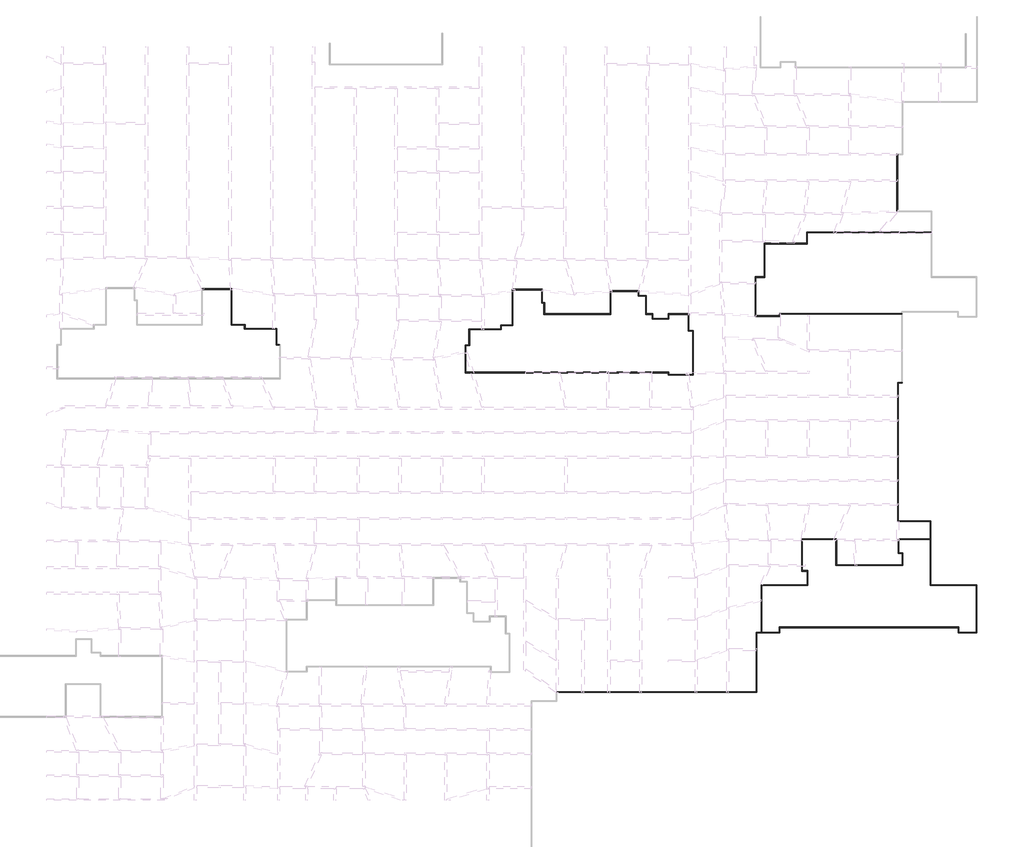
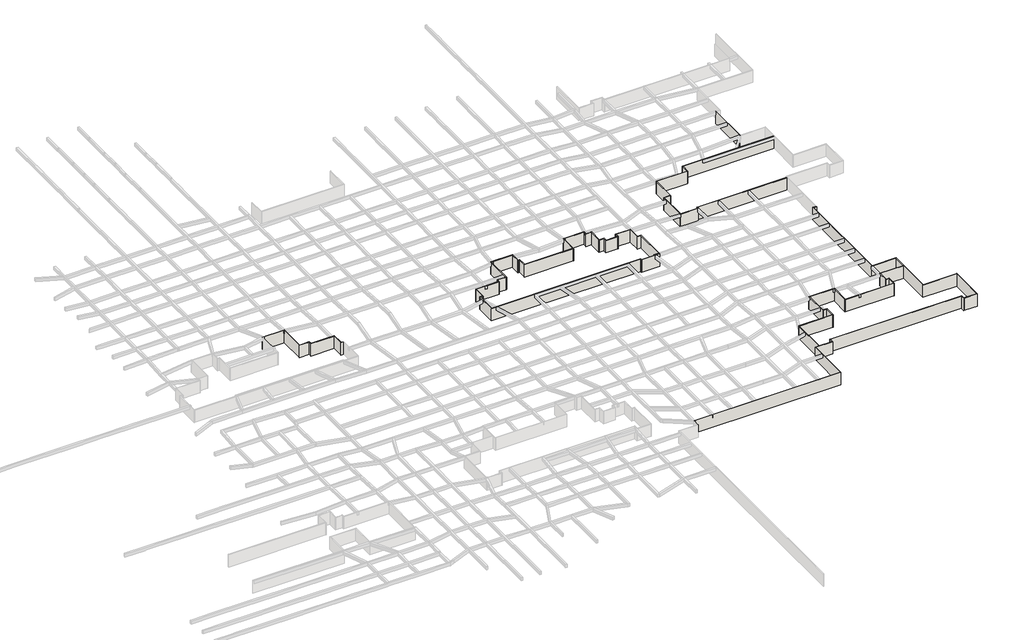
# One storey, part 4 of 45: 70 walls.
"""IFC4 building model written with IfcOpenShell, lengths in millimetres."""

from ifc_helpers import new_model, si_unit, origin, origin_with_axes, place, context, project, spatial, polyline, outline, extrude, faceted_brep, element, save

model = new_model("IFC4")

# Units and contexts
model_context = context("Model", 3, world=origin())
ifc_project = project(units=[si_unit("LENGTHUNIT", "METRE", prefix="MILLI")], contexts=[model_context])

# Site, building, storey
site = spatial("IfcSite", under=ifc_project)
building = spatial("IfcBuilding", under=site)
storey = spatial("IfcBuildingStorey", under=building, Name="户型图", Elevation=0.0)

# Walls
placement = place(None, origin())
element("IfcWall", 1, ObjectType="所有墙体", at=placement, inside=storey, context=model_context, shape_type="Brep", body=[
    faceted_brep([(-180.5216564, -109988.0123265, 0.0), (37119.4783436, -109988.0123265, 0.0), (37119.4783436, -109988.0123265, 3300.0), (-180.5216564, -109988.0123265, 3300.0), (-180.5216564, -109868.0123265, 0.0), (-180.5216564, -109868.0123265, 3300.0), (36999.4783436, -109868.0123265, 3300.0), (37119.4783436, -109868.0123265, 3300.0), (37119.4783436, -109868.0123265, 0.0), (36999.4783436, -109868.0123265, 0.0)], [[[0, 1, 2, 3]], [[4, 5, 6, 7, 8, 9]], [[1, 0, 4, 9, 8]], [[3, 2, 7, 6, 5]], [[0, 3, 5, 4]], [[2, 1, 8, 7]]]),
])
element("IfcWall", 2, ObjectType="所有墙体", at=placement, inside=storey, context=model_context, shape_type="Brep", body=[
    faceted_brep([(37119.4783436, -109868.0123265, 0.0), (37119.4783436, -98888.0123265, 0.0), (37119.4783436, -98768.0123265, 0.0), (37119.4783436, -98768.0123265, 3300.0), (37119.4783436, -98888.0123265, 3300.0), (37119.4783436, -109868.0123265, 3300.0), (36999.4783436, -109868.0123265, 0.0), (36999.4783436, -109868.0123265, 3300.0), (36999.4783436, -98768.0123265, 3300.0), (36999.4783436, -98768.0123265, 0.0)], [[[0, 1, 2, 3, 4, 5]], [[6, 7, 8, 9]], [[2, 1, 0, 6, 9]], [[5, 4, 3, 8, 7]], [[0, 5, 7, 6]], [[3, 2, 9, 8]]]),
])
element("IfcWall", 3, ObjectType="所有墙体", at=placement, inside=storey, context=model_context, shape_type="Brep", body=[
    faceted_brep([(37119.4783436, -98888.0123265, 0.0), (41419.4783436, -98888.0123265, 0.0), (41419.4783436, -98888.0123265, 3300.0), (37119.4783436, -98888.0123265, 3300.0), (37119.4783436, -98768.0123265, 0.0), (37119.4783436, -98768.0123265, 3300.0), (37945.7968791, -98768.0123265, 3300.0), (38065.7968791, -98768.0123265, 3300.0), (41299.4783436, -98768.0123265, 3300.0), (41419.4783436, -98768.0123265, 3300.0), (41419.4783436, -98768.0123265, 0.0), (41299.4783436, -98768.0123265, 0.0), (38065.7968791, -98768.0123265, 0.0), (37945.7968791, -98768.0123265, 0.0)], [[[0, 1, 2, 3]], [[4, 5, 6, 7, 8, 9, 10, 11, 12, 13]], [[1, 0, 4, 13, 12, 11, 10]], [[3, 2, 9, 8, 7, 6, 5]], [[0, 3, 5, 4]], [[2, 1, 10, 9]]]),
])
element("IfcWall", 4, ObjectType="所有墙体", at=placement, inside=storey, context=model_context, shape_type="Brep", body=[
    faceted_brep([(41419.4783436, -98768.0123265, 0.0), (41419.4783436, -97888.0123265, 0.0), (41419.4783436, -97768.0123265, 0.0), (41419.4783436, -97768.0123265, 3300.0), (41419.4783436, -97888.0123265, 3300.0), (41419.4783436, -98768.0123265, 3300.0), (41299.4783436, -98768.0123265, 0.0), (41299.4783436, -98768.0123265, 3300.0), (41299.4783436, -97768.0123265, 3300.0), (41299.4783436, -97768.0123265, 0.0)], [[[0, 1, 2, 3, 4, 5]], [[6, 7, 8, 9]], [[2, 1, 0, 6, 9]], [[5, 4, 3, 8, 7]], [[0, 5, 7, 6]], [[3, 2, 9, 8]]]),
])
element("IfcWall", 5, ObjectType="所有墙体", at=placement, inside=storey, context=model_context, shape_type="Brep", body=[
    faceted_brep([(41419.4783436, -97888.0123265, 0.0), (74699.4783436, -97888.0123265, 0.0), (74819.4783436, -97888.0123265, 0.0), (74819.4783436, -97888.0123265, 3300.0), (74699.4783436, -97888.0123265, 3300.0), (41419.4783436, -97888.0123265, 3300.0), (41419.4783436, -97768.0123265, 0.0), (41419.4783436, -97768.0123265, 3300.0), (74819.4783436, -97768.0123265, 3300.0), (74819.4783436, -97768.0123265, 0.0)], [[[0, 1, 2, 3, 4, 5]], [[6, 7, 8, 9]], [[2, 1, 0, 6, 9]], [[5, 4, 3, 8, 7]], [[0, 5, 7, 6]], [[3, 2, 9, 8]]]),
])
element("IfcWall", 6, ObjectType="所有墙体", at=placement, inside=storey, context=model_context, shape_type="Brep", body=[
    faceted_brep([(74699.4783436, -97888.0123265, 0.0), (74699.4783436, -98888.0123265, 0.0), (74699.4783436, -98888.0123265, 3300.0), (74699.4783436, -97888.0123265, 3300.0), (74819.4783436, -97888.0123265, 0.0), (74819.4783436, -97888.0123265, 3300.0), (74819.4783436, -98768.0123265, 3300.0), (74819.4783436, -98888.0123265, 3300.0), (74819.4783436, -98888.0123265, 0.0), (74819.4783436, -98768.0123265, 0.0)], [[[0, 1, 2, 3]], [[4, 5, 6, 7, 8, 9]], [[1, 0, 4, 9, 8]], [[3, 2, 7, 6, 5]], [[0, 3, 5, 4]], [[2, 1, 8, 7]]]),
])
element("IfcWall", 7, ObjectType="所有墙体", at=placement, inside=storey, context=model_context, shape_type="Brep", body=[
    faceted_brep([(74819.4783436, -98888.0123265, 0.0), (78219.4783436, -98888.0123265, 0.0), (78219.4783436, -98888.0123265, 3300.0), (74819.4783436, -98888.0123265, 3300.0), (74819.4783436, -98768.0123265, 0.0), (74819.4783436, -98768.0123265, 3300.0), (78099.4783436, -98768.0123265, 3300.0), (78219.4783436, -98768.0123265, 3300.0), (78219.4783436, -98768.0123265, 0.0), (78099.4783436, -98768.0123265, 0.0)], [[[0, 1, 2, 3]], [[4, 5, 6, 7, 8, 9]], [[1, 0, 4, 9, 8]], [[3, 2, 7, 6, 5]], [[0, 3, 5, 4]], [[2, 1, 8, 7]]]),
])
element("IfcWall", 8, ObjectType="所有墙体", at=placement, inside=storey, context=model_context, shape_type="Brep", body=[
    faceted_brep([(78219.4783436, -98768.0123265, 0.0), (78219.4783436, -89868.0123265, 0.0), (78219.4783436, -89868.0123265, 3300.0), (78219.4783436, -98768.0123265, 3300.0), (78099.4783436, -98768.0123265, 0.0), (78099.4783436, -98768.0123265, 3300.0), (78099.4783436, -89988.0123265, 3300.0), (78099.4783436, -89868.0123265, 3300.0), (78099.4783436, -89868.0123265, 0.0), (78099.4783436, -89988.0123265, 0.0)], [[[0, 1, 2, 3]], [[4, 5, 6, 7, 8, 9]], [[1, 0, 4, 9, 8]], [[3, 2, 7, 6, 5]], [[0, 3, 5, 4]], [[2, 1, 8, 7]]]),
])
element("IfcWall", 9, ObjectType="所有墙体", at=placement, inside=storey, context=model_context, shape_type="Brep", body=[
    faceted_brep([(78099.4783436, -89868.0123265, 0.0), (69619.4783436, -89868.0123265, 0.0), (69499.4783436, -89868.0123265, 0.0), (69499.4783436, -89868.0123265, 3300.0), (69619.4783436, -89868.0123265, 3300.0), (78099.4783436, -89868.0123265, 3300.0), (78099.4783436, -89988.0123265, 0.0), (78099.4783436, -89988.0123265, 3300.0), (69499.4783436, -89988.0123265, 3300.0), (69499.4783436, -89988.0123265, 0.0)], [[[0, 1, 2, 3, 4, 5]], [[6, 7, 8, 9]], [[2, 1, 0, 6, 9]], [[5, 4, 3, 8, 7]], [[0, 5, 7, 6]], [[3, 2, 9, 8]]]),
])
element("IfcWall", 10, ObjectType="所有墙体", at=placement, inside=storey, context=model_context, shape_type="Brep", body=[
    faceted_brep([(69619.4783436, -89868.0123265, 0.0), (69619.4783436, -77968.0123265, 0.0), (69619.4783436, -77968.0123265, 3300.0), (69619.4783436, -89868.0123265, 3300.0), (69499.4783436, -89868.0123265, 0.0), (69499.4783436, -89868.0123265, 3300.0), (69499.4783436, -81448.0123265, 3300.0), (69499.4783436, -81328.0123265, 3300.0), (69499.4783436, -78088.0123265, 3300.0), (69499.4783436, -77968.0123265, 3300.0), (69499.4783436, -77968.0123265, 0.0), (69499.4783436, -78088.0123265, 0.0), (69499.4783436, -81328.0123265, 0.0), (69499.4783436, -81448.0123265, 0.0)], [[[0, 1, 2, 3]], [[4, 5, 6, 7, 8, 9, 10, 11, 12, 13]], [[1, 0, 4, 13, 12, 11, 10]], [[3, 2, 9, 8, 7, 6, 5]], [[0, 3, 5, 4]], [[2, 1, 10, 9]]]),
])
element("IfcWall", 11, ObjectType="所有墙体", at=placement, inside=storey, context=model_context, shape_type="Brep", body=[
    faceted_brep([(69499.4783436, -77968.0123265, 0.0), (63519.4783436, -77968.0123265, 0.0), (63399.4783436, -77968.0123265, 0.0), (63399.4783436, -77968.0123265, 3300.0), (63519.4783436, -77968.0123265, 3300.0), (69499.4783436, -77968.0123265, 3300.0), (69499.4783436, -78088.0123265, 0.0), (69499.4783436, -78088.0123265, 3300.0), (63399.4783436, -78088.0123265, 3300.0), (63399.4783436, -78088.0123265, 0.0)], [[[0, 1, 2, 3, 4, 5]], [[6, 7, 8, 9]], [[2, 1, 0, 6, 9]], [[5, 4, 3, 8, 7]], [[0, 5, 7, 6]], [[3, 2, 9, 8]]]),
])
element("IfcWall", 12, ObjectType="所有墙体", at=placement, inside=storey, context=model_context, shape_type="Brep", body=[
    faceted_brep([(63519.4783436, -77968.0123265, 0.0), (63519.4783436, -52188.0123265, 0.0), (63519.4783436, -52068.0123265, 0.0), (63519.4783436, -52068.0123265, 3300.0), (63519.4783436, -52188.0123265, 3300.0), (63519.4783436, -77968.0123265, 3300.0), (63399.4783436, -77968.0123265, 0.0), (63399.4783436, -77968.0123265, 3300.0), (63399.4783436, -52068.0123265, 3300.0), (63399.4783436, -52068.0123265, 0.0)], [[[0, 1, 2, 3, 4, 5]], [[6, 7, 8, 9]], [[2, 1, 0, 6, 9]], [[5, 4, 3, 8, 7]], [[0, 5, 7, 6]], [[3, 2, 9, 8]]]),
])
element("IfcWall", 13, ObjectType="所有墙体", at=placement, inside=storey, context=model_context, shape_type="Brep", body=[
    faceted_brep([(63519.4783436, -52188.0123265, 0.0), (64319.4783436, -52188.0123265, 0.0), (64319.4783436, -52188.0123265, 3300.0), (63519.4783436, -52188.0123265, 3300.0), (63519.4783436, -52068.0123265, 0.0), (63519.4783436, -52068.0123265, 3300.0), (64199.4783436, -52068.0123265, 3300.0), (64319.4783436, -52068.0123265, 3300.0), (64319.4783436, -52068.0123265, 0.0), (64199.4783436, -52068.0123265, 0.0)], [[[0, 1, 2, 3]], [[4, 5, 6, 7, 8, 9]], [[1, 0, 4, 9, 8]], [[3, 2, 7, 6, 5]], [[0, 3, 5, 4]], [[2, 1, 8, 7]]]),
])
element("IfcWall", 14, ObjectType="所有墙体", at=placement, inside=storey, context=model_context, shape_type="Brep", body=[
    faceted_brep([(63419.4783436, -20068.0123265, 0.0), (63419.4783436, -9588.0123265, 0.0), (63419.4783436, -9468.0123265, 0.0), (63419.4783436, -9468.0123265, 3300.0), (63419.4783436, -9588.0123265, 3300.0), (63419.4783436, -20068.0123265, 3300.0), (63299.4783436, -20068.0123265, 0.0), (63299.4783436, -20068.0123265, 3300.0), (63299.4783436, -9468.0123265, 3300.0), (63299.4783436, -9468.0123265, 0.0)], [[[0, 1, 2, 3, 4, 5]], [[6, 7, 8, 9]], [[2, 1, 0, 6, 9]], [[5, 4, 3, 8, 7]], [[0, 5, 7, 6]], [[3, 2, 9, 8]]]),
])
element("IfcWall", 15, ObjectType="所有墙体", at=placement, inside=storey, context=model_context, shape_type="Brep", body=[
    faceted_brep([(69699.4783436, -24010.6851163, 0.0), (46417.7693877, -24010.6851163, 0.0), (46417.7693877, -24010.6851163, 3300.0), (69699.4783436, -24010.6851163, 3300.0), (69699.4783436, -24130.6851163, 0.0), (69699.4783436, -24130.6851163, 3300.0), (46537.7693877, -24130.6851163, 3300.0), (46417.7693877, -24130.6851163, 3300.0), (46417.7693877, -24130.6851163, 0.0), (46537.7693877, -24130.6851163, 0.0)], [[[0, 1, 2, 3]], [[4, 5, 6, 7, 8, 9]], [[1, 0, 4, 9, 8]], [[3, 2, 7, 6, 5]], [[2, 1, 8, 7]], [[0, 3, 5, 4]]]),
])
element("IfcWall", 16, ObjectType="所有墙体", at=placement, inside=storey, context=model_context, shape_type="Brep", body=[
    faceted_brep([(46417.7693877, -24130.6851163, 0.0), (46417.7693877, -26110.6851163, 0.0), (46417.7693877, -26230.6851163, 0.0), (46417.7693877, -26230.6851163, 3300.0), (46417.7693877, -26110.6851163, 3300.0), (46417.7693877, -24130.6851163, 3300.0), (46537.7693877, -24130.6851163, 0.0), (46537.7693877, -24130.6851163, 3300.0), (46537.7693877, -26230.6851163, 3300.0), (46537.7693877, -26230.6851163, 0.0)], [[[0, 1, 2, 3, 4, 5]], [[6, 7, 8, 9]], [[2, 1, 0, 6, 9]], [[5, 4, 3, 8, 7]], [[0, 5, 7, 6]], [[3, 2, 9, 8]]]),
])
element("IfcWall", 17, ObjectType="所有墙体", at=placement, inside=storey, context=model_context, shape_type="Brep", body=[
    faceted_brep([(46417.7693877, -26110.6851163, 0.0), (38517.7693877, -26110.6851163, 0.0), (38517.7693877, -26110.6851163, 3300.0), (46417.7693877, -26110.6851163, 3300.0), (46417.7693877, -26230.6851163, 0.0), (46417.7693877, -26230.6851163, 3300.0), (38637.7693877, -26230.6851163, 3300.0), (38517.7693877, -26230.6851163, 3300.0), (38517.7693877, -26230.6851163, 0.0), (38637.7693877, -26230.6851163, 0.0)], [[[0, 1, 2, 3]], [[4, 5, 6, 7, 8, 9]], [[1, 0, 4, 9, 8]], [[3, 2, 7, 6, 5]], [[0, 3, 5, 4]], [[2, 1, 8, 7]]]),
])
element("IfcWall", 18, ObjectType="所有墙体", at=placement, inside=storey, context=model_context, shape_type="Brep", body=[
    faceted_brep([(38517.7693877, -26230.6851163, 0.0), (38517.7693877, -32368.0123265, 0.0), (38517.7693877, -32488.0123265, 0.0), (38517.7693877, -32488.0123265, 3300.0), (38517.7693877, -32368.0123265, 3300.0), (38517.7693877, -26230.6851163, 3300.0), (38637.7693877, -26230.6851163, 0.0), (38637.7693877, -26230.6851163, 3300.0), (38637.7693877, -32488.0123265, 3300.0), (38637.7693877, -32488.0123265, 0.0)], [[[0, 1, 2, 3, 4, 5]], [[6, 7, 8, 9]], [[2, 1, 0, 6, 9]], [[5, 4, 3, 8, 7]], [[0, 5, 7, 6]], [[3, 2, 9, 8]]]),
])
element("IfcWall", 19, ObjectType="所有墙体", at=placement, inside=storey, context=model_context, shape_type="Brep", body=[
    faceted_brep([(38517.7693877, -32368.0123265, 0.0), (36817.7693877, -32368.0123265, 0.0), (36817.7693877, -32368.0123265, 3300.0), (38517.7693877, -32368.0123265, 3300.0), (38517.7693877, -32488.0123265, 0.0), (38517.7693877, -32488.0123265, 3300.0), (36937.7693877, -32488.0123265, 3300.0), (36817.7693877, -32488.0123265, 3300.0), (36817.7693877, -32488.0123265, 0.0), (36937.7693877, -32488.0123265, 0.0)], [[[0, 1, 2, 3]], [[4, 5, 6, 7, 8, 9]], [[1, 0, 4, 9, 8]], [[3, 2, 7, 6, 5]], [[0, 3, 5, 4]], [[2, 1, 8, 7]]]),
])
element("IfcWall", 20, ObjectType="所有墙体", at=placement, inside=storey, context=model_context, shape_type="Brep", body=[
    faceted_brep([(36817.7693877, -32488.0123265, 0.0), (36817.7693877, -39754.4925986, 0.0), (36817.7693877, -39754.4925986, 3300.0), (36817.7693877, -32488.0123265, 3300.0), (36937.7693877, -32488.0123265, 0.0), (36937.7693877, -32488.0123265, 3300.0), (36937.7693877, -39634.4925986, 3300.0), (36937.7693877, -39754.4925986, 3300.0), (36937.7693877, -39754.4925986, 0.0), (36937.7693877, -39634.4925986, 0.0)], [[[0, 1, 2, 3]], [[4, 5, 6, 7, 8, 9]], [[1, 0, 4, 9, 8]], [[3, 2, 7, 6, 5]], [[0, 3, 5, 4]], [[2, 1, 8, 7]]]),
])
element("IfcWall", 21, ObjectType="所有墙体", at=placement, inside=storey, context=model_context, shape_type="Brep", body=[
    faceted_brep([(36937.7693877, -39754.4925986, 0.0), (41406.5225603, -39754.4925986, 0.0), (41406.5225603, -39754.4925986, 3300.0), (36937.7693877, -39754.4925986, 3300.0), (36937.7693877, -39634.4925986, 0.0), (36937.7693877, -39634.4925986, 3300.0), (41286.5225603, -39634.4925986, 3300.0), (41406.5225603, -39634.4925986, 3300.0), (41406.5225603, -39634.4925986, 0.0), (41286.5225603, -39634.4925986, 0.0)], [[[0, 1, 2, 3]], [[4, 5, 6, 7, 8, 9]], [[1, 0, 4, 9, 8]], [[3, 2, 7, 6, 5]], [[0, 3, 5, 4]], [[2, 1, 8, 7]]]),
])
element("IfcWall", 22, ObjectType="所有墙体", at=placement, inside=storey, context=model_context, shape_type="Brep", body=[
    faceted_brep([(41406.5225603, -39634.4925986, 0.0), (41406.5225603, -39338.8304418, 0.0), (41406.5225603, -39218.8304418, 0.0), (41406.5225603, -39218.8304418, 3300.0), (41406.5225603, -39338.8304418, 3300.0), (41406.5225603, -39634.4925986, 3300.0), (41286.5225603, -39634.4925986, 0.0), (41286.5225603, -39634.4925986, 3300.0), (41286.5225603, -39218.8304418, 3300.0), (41286.5225603, -39218.8304418, 0.0)], [[[0, 1, 2, 3, 4, 5]], [[6, 7, 8, 9]], [[2, 1, 0, 6, 9]], [[5, 4, 3, 8, 7]], [[0, 5, 7, 6]], [[3, 2, 9, 8]]]),
])
element("IfcWall", 23, ObjectType="所有墙体", at=placement, inside=storey, context=model_context, shape_type="SweptSolid", body=[
    extrude(outline(polyline([(64199.4783436, -39338.8304418), (41406.5225603, -39338.8304418), (41406.5225603, -39218.8304418), (64199.4783436, -39218.8304418), (64199.4783436, -39338.8304418)])), origin_with_axes(), (0.0, 0.0, 1.0), 3300.0),
])
element("IfcWall", 24, ObjectType="所有墙体", at=placement, inside=storey, context=model_context, shape_type="Brep", body=[
    faceted_brep([(-17290.1931615, -50294.901078, 0.0), (20578.0119922, -50294.901078, 0.0), (20698.0119922, -50294.901078, 0.0), (20698.0119922, -50294.901078, 3300.0), (20578.0119922, -50294.901078, 3300.0), (-17290.1931615, -50294.901078, 3300.0), (-17290.1931615, -50174.901078, 0.0), (-17290.1931615, -50174.901078, 3300.0), (-17170.1931615, -50174.901078, 3300.0), (20698.0119922, -50174.901078, 3300.0), (20698.0119922, -50174.901078, 0.0), (-17170.1931615, -50174.901078, 0.0)], [[[0, 1, 2, 3, 4, 5]], [[6, 7, 8, 9, 10, 11]], [[2, 1, 0, 6, 11, 10]], [[5, 4, 3, 9, 8, 7]], [[3, 2, 10, 9]], [[0, 5, 7, 6]]]),
])
element("IfcWall", 25, ObjectType="所有墙体", at=placement, inside=storey, context=model_context, shape_type="Brep", body=[
    faceted_brep([(20578.0119922, -50294.901078, 0.0), (20578.0119922, -50694.901078, 0.0), (20578.0119922, -50694.901078, 3300.0), (20578.0119922, -50294.901078, 3300.0), (20698.0119922, -50294.901078, 0.0), (20698.0119922, -50294.901078, 3300.0), (20698.0119922, -50574.901078, 3300.0), (20698.0119922, -50694.901078, 3300.0), (20698.0119922, -50694.901078, 0.0), (20698.0119922, -50574.901078, 0.0)], [[[0, 1, 2, 3]], [[4, 5, 6, 7, 8, 9]], [[1, 0, 4, 9, 8]], [[3, 2, 7, 6, 5]], [[0, 3, 5, 4]], [[2, 1, 8, 7]]]),
])
element("IfcWall", 26, ObjectType="所有墙体", at=placement, inside=storey, context=model_context, shape_type="Brep", body=[
    faceted_brep([(20698.0119922, -50694.901078, 0.0), (25318.1490674, -50694.901078, 0.0), (25318.1490674, -50694.901078, 3300.0), (20698.0119922, -50694.901078, 3300.0), (20698.0119922, -50574.901078, 0.0), (20698.0119922, -50574.901078, 3300.0), (25198.1490674, -50574.901078, 3300.0), (25318.1490674, -50574.901078, 3300.0), (25318.1490674, -50574.901078, 0.0), (25198.1490674, -50574.901078, 0.0)], [[[0, 1, 2, 3]], [[4, 5, 6, 7, 8, 9]], [[1, 0, 4, 9, 8]], [[3, 2, 7, 6, 5]], [[0, 3, 5, 4]], [[2, 1, 8, 7]]]),
])
element("IfcWall", 27, ObjectType="所有墙体", at=placement, inside=storey, context=model_context, shape_type="Brep", body=[
    faceted_brep([(25318.1490674, -50574.901078, 0.0), (25318.1490674, -42374.901078, 0.0), (25318.1490674, -42374.901078, 3300.0), (25318.1490674, -50574.901078, 3300.0), (25198.1490674, -50574.901078, 0.0), (25198.1490674, -50574.901078, 3300.0), (25198.1490674, -42494.901078, 3300.0), (25198.1490674, -42374.901078, 3300.0), (25198.1490674, -42374.901078, 0.0), (25198.1490674, -42494.901078, 0.0)], [[[0, 1, 2, 3]], [[4, 5, 6, 7, 8, 9]], [[1, 0, 4, 9, 8]], [[3, 2, 7, 6, 5]], [[0, 3, 5, 4]], [[2, 1, 8, 7]]]),
])
element("IfcWall", 28, ObjectType="所有墙体", at=placement, inside=storey, context=model_context, shape_type="Brep", body=[
    faceted_brep([(25198.1490674, -42374.901078, 0.0), (24418.1490674, -42374.901078, 0.0), (24298.1490674, -42374.901078, 0.0), (24298.1490674, -42374.901078, 3300.0), (24418.1490674, -42374.901078, 3300.0), (25198.1490674, -42374.901078, 3300.0), (25198.1490674, -42494.901078, 0.0), (25198.1490674, -42494.901078, 3300.0), (24298.1490674, -42494.901078, 3300.0), (24298.1490674, -42494.901078, 0.0)], [[[0, 1, 2, 3, 4, 5]], [[6, 7, 8, 9]], [[2, 1, 0, 6, 9]], [[5, 4, 3, 8, 7]], [[0, 5, 7, 6]], [[3, 2, 9, 8]]]),
])
element("IfcWall", 29, ObjectType="所有墙体", at=placement, inside=storey, context=model_context, shape_type="Brep", body=[
    faceted_brep([(24418.1490674, -42374.901078, 0.0), (24418.1490674, -39274.901078, 0.0), (24418.1490674, -39274.901078, 3300.0), (24418.1490674, -42374.901078, 3300.0), (24298.1490674, -42374.901078, 0.0), (24298.1490674, -42374.901078, 3300.0), (24298.1490674, -39394.901078, 3300.0), (24298.1490674, -39274.901078, 3300.0), (24298.1490674, -39274.901078, 0.0), (24298.1490674, -39394.901078, 0.0)], [[[0, 1, 2, 3]], [[4, 5, 6, 7, 8, 9]], [[1, 0, 4, 9, 8]], [[3, 2, 7, 6, 5]], [[0, 3, 5, 4]], [[2, 1, 8, 7]]]),
])
element("IfcWall", 30, ObjectType="所有墙体", at=placement, inside=storey, context=model_context, shape_type="Brep", body=[
    faceted_brep([(24298.1490674, -39274.901078, 0.0), (20598.1490674, -39274.901078, 0.0), (20598.1490674, -39274.901078, 3300.0), (24298.1490674, -39274.901078, 3300.0), (24298.1490674, -39394.901078, 0.0), (24298.1490674, -39394.901078, 3300.0), (20718.1490674, -39394.901078, 3300.0), (20598.1490674, -39394.901078, 3300.0), (20598.1490674, -39394.901078, 0.0), (20718.1490674, -39394.901078, 0.0)], [[[0, 1, 2, 3]], [[4, 5, 6, 7, 8, 9]], [[1, 0, 4, 9, 8]], [[3, 2, 7, 6, 5]], [[0, 3, 5, 4]], [[2, 1, 8, 7]]]),
])
element("IfcWall", 31, ObjectType="所有墙体", at=placement, inside=storey, context=model_context, shape_type="Brep", body=[
    faceted_brep([(20598.1490674, -39394.901078, 0.0), (20598.1490674, -40174.901078, 0.0), (20598.1490674, -40294.901078, 0.0), (20598.1490674, -40294.901078, 3300.0), (20598.1490674, -40174.901078, 3300.0), (20598.1490674, -39394.901078, 3300.0), (20718.1490674, -39394.901078, 0.0), (20718.1490674, -39394.901078, 3300.0), (20718.1490674, -40294.901078, 3300.0), (20718.1490674, -40294.901078, 0.0)], [[[0, 1, 2, 3, 4, 5]], [[6, 7, 8, 9]], [[2, 1, 0, 6, 9]], [[5, 4, 3, 8, 7]], [[0, 5, 7, 6]], [[3, 2, 9, 8]]]),
])
element("IfcWall", 32, ObjectType="所有墙体", at=placement, inside=storey, context=model_context, shape_type="Brep", body=[
    faceted_brep([(20598.1490674, -40174.901078, 0.0), (17718.1490674, -40174.901078, 0.0), (17598.1490674, -40174.901078, 0.0), (17598.1490674, -40174.901078, 3300.0), (17718.1490674, -40174.901078, 3300.0), (20598.1490674, -40174.901078, 3300.0), (20598.1490674, -40294.901078, 0.0), (20598.1490674, -40294.901078, 3300.0), (17598.1490674, -40294.901078, 3300.0), (17598.1490674, -40294.901078, 0.0)], [[[0, 1, 2, 3, 4, 5]], [[6, 7, 8, 9]], [[2, 1, 0, 6, 9]], [[5, 4, 3, 8, 7]], [[0, 5, 7, 6]], [[3, 2, 9, 8]]]),
])
element("IfcWall", 33, ObjectType="所有墙体", at=placement, inside=storey, context=model_context, shape_type="Brep", body=[
    faceted_brep([(17718.1490674, -40174.901078, 0.0), (17718.1490674, -39274.901078, 0.0), (17718.1490674, -39274.901078, 3300.0), (17718.1490674, -40174.901078, 3300.0), (17598.1490674, -40174.901078, 0.0), (17598.1490674, -40174.901078, 3300.0), (17598.1490674, -39394.901078, 3300.0), (17598.1490674, -39274.901078, 3300.0), (17598.1490674, -39274.901078, 0.0), (17598.1490674, -39394.901078, 0.0)], [[[0, 1, 2, 3]], [[4, 5, 6, 7, 8, 9]], [[1, 0, 4, 9, 8]], [[3, 2, 7, 6, 5]], [[0, 3, 5, 4]], [[2, 1, 8, 7]]]),
])
element("IfcWall", 34, ObjectType="所有墙体", at=placement, inside=storey, context=model_context, shape_type="Brep", body=[
    faceted_brep([(17598.1490674, -39274.901078, 0.0), (16518.1490674, -39274.901078, 0.0), (16398.1490674, -39274.901078, 0.0), (16398.1490674, -39274.901078, 3300.0), (16518.1490674, -39274.901078, 3300.0), (17598.1490674, -39274.901078, 3300.0), (17598.1490674, -39394.901078, 0.0), (17598.1490674, -39394.901078, 3300.0), (16398.1490674, -39394.901078, 3300.0), (16398.1490674, -39394.901078, 0.0)], [[[0, 1, 2, 3, 4, 5]], [[6, 7, 8, 9]], [[2, 1, 0, 6, 9]], [[5, 4, 3, 8, 7]], [[0, 5, 7, 6]], [[3, 2, 9, 8]]]),
])
element("IfcWall", 35, ObjectType="所有墙体", at=placement, inside=storey, context=model_context, shape_type="Brep", body=[
    faceted_brep([(16518.1490674, -39274.901078, 0.0), (16518.1490674, -35874.901078, 0.0), (16518.1490674, -35874.901078, 3300.0), (16518.1490674, -39274.901078, 3300.0), (16398.1490674, -39274.901078, 0.0), (16398.1490674, -39274.901078, 3300.0), (16398.1490674, -35994.901078, 3300.0), (16398.1490674, -35874.901078, 3300.0), (16398.1490674, -35874.901078, 0.0), (16398.1490674, -35994.901078, 0.0)], [[[0, 1, 2, 3]], [[4, 5, 6, 7, 8, 9]], [[1, 0, 4, 9, 8]], [[3, 2, 7, 6, 5]], [[0, 3, 5, 4]], [[2, 1, 8, 7]]]),
])
element("IfcWall", 36, ObjectType="所有墙体", at=placement, inside=storey, context=model_context, shape_type="Brep", body=[
    faceted_brep([(16398.1490674, -35874.901078, 0.0), (15118.1490674, -35874.901078, 0.0), (14998.1490674, -35874.901078, 0.0), (14998.1490674, -35874.901078, 3300.0), (15118.1490674, -35874.901078, 3300.0), (16398.1490674, -35874.901078, 3300.0), (16398.1490674, -35994.901078, 0.0), (16398.1490674, -35994.901078, 3300.0), (14998.1490674, -35994.901078, 3300.0), (14998.1490674, -35994.901078, 0.0)], [[[0, 1, 2, 3, 4, 5]], [[6, 7, 8, 9]], [[2, 1, 0, 6, 9]], [[5, 4, 3, 8, 7]], [[0, 5, 7, 6]], [[3, 2, 9, 8]]]),
])
element("IfcWall", 37, ObjectType="所有墙体", at=placement, inside=storey, context=model_context, shape_type="Brep", body=[
    faceted_brep([(15118.1490674, -35874.901078, 0.0), (15118.1490674, -34974.901078, 0.0), (15118.1490674, -34974.901078, 3300.0), (15118.1490674, -35874.901078, 3300.0), (14998.1490674, -35874.901078, 0.0), (14998.1490674, -35874.901078, 3300.0), (14998.1490674, -35094.901078, 3300.0), (14998.1490674, -34974.901078, 3300.0), (14998.1490674, -34974.901078, 0.0), (14998.1490674, -35094.901078, 0.0)], [[[0, 1, 2, 3]], [[4, 5, 6, 7, 8, 9]], [[1, 0, 4, 9, 8]], [[3, 2, 7, 6, 5]], [[0, 3, 5, 4]], [[2, 1, 8, 7]]]),
])
element("IfcWall", 38, ObjectType="所有墙体", at=placement, inside=storey, context=model_context, shape_type="Brep", body=[
    faceted_brep([(14998.1490674, -34974.901078, 0.0), (9798.1490674, -34974.901078, 0.0), (9798.1490674, -34974.901078, 3300.0), (14998.1490674, -34974.901078, 3300.0), (14998.1490674, -35094.901078, 0.0), (14998.1490674, -35094.901078, 3300.0), (9918.1490674, -35094.901078, 3300.0), (9798.1490674, -35094.901078, 3300.0), (9798.1490674, -35094.901078, 0.0), (9918.1490674, -35094.901078, 0.0)], [[[0, 1, 2, 3]], [[4, 5, 6, 7, 8, 9]], [[1, 0, 4, 9, 8]], [[3, 2, 7, 6, 5]], [[0, 3, 5, 4]], [[2, 1, 8, 7]]]),
])
element("IfcWall", 39, ObjectType="所有墙体", at=placement, inside=storey, context=model_context, shape_type="Brep", body=[
    faceted_brep([(9798.1490674, -35094.901078, 0.0), (9798.1490674, -39274.901078, 0.0), (9798.1490674, -39394.901078, 0.0), (9798.1490674, -39394.901078, 3300.0), (9798.1490674, -39274.901078, 3300.0), (9798.1490674, -35094.901078, 3300.0), (9918.1490674, -35094.901078, 0.0), (9918.1490674, -35094.901078, 3300.0), (9918.1490674, -39394.901078, 3300.0), (9918.1490674, -39394.901078, 0.0)], [[[0, 1, 2, 3, 4, 5]], [[6, 7, 8, 9]], [[2, 1, 0, 6, 9]], [[5, 4, 3, 8, 7]], [[0, 5, 7, 6]], [[3, 2, 9, 8]]]),
])
element("IfcWall", 40, ObjectType="所有墙体", at=placement, inside=storey, context=model_context, shape_type="Brep", body=[
    faceted_brep([(9798.1490674, -39274.901078, 0.0), (-2481.8509326, -39274.901078, 0.0), (-2601.8509326, -39274.901078, 0.0), (-2601.8509326, -39274.901078, 3300.0), (-2481.8509326, -39274.901078, 3300.0), (9798.1490674, -39274.901078, 3300.0), (9798.1490674, -39394.901078, 0.0), (9798.1490674, -39394.901078, 3300.0), (-2601.8509326, -39394.901078, 3300.0), (-2601.8509326, -39394.901078, 0.0)], [[[0, 1, 2, 3, 4, 5]], [[6, 7, 8, 9]], [[2, 1, 0, 6, 9]], [[5, 4, 3, 8, 7]], [[0, 5, 7, 6]], [[3, 2, 9, 8]]]),
])
element("IfcWall", 41, ObjectType="所有墙体", at=placement, inside=storey, context=model_context, shape_type="Brep", body=[
    faceted_brep([(-2481.8509326, -39274.901078, 0.0), (-2481.8509326, -37174.901078, 0.0), (-2481.8509326, -37174.901078, 3300.0), (-2481.8509326, -39274.901078, 3300.0), (-2601.8509326, -39274.901078, 0.0), (-2601.8509326, -39274.901078, 3300.0), (-2601.8509326, -37294.901078, 3300.0), (-2601.8509326, -37174.901078, 3300.0), (-2601.8509326, -37174.901078, 0.0), (-2601.8509326, -37294.901078, 0.0)], [[[0, 1, 2, 3]], [[4, 5, 6, 7, 8, 9]], [[1, 0, 4, 9, 8]], [[3, 2, 7, 6, 5]], [[0, 3, 5, 4]], [[2, 1, 8, 7]]]),
])
element("IfcWall", 42, ObjectType="所有墙体", at=placement, inside=storey, context=model_context, shape_type="Brep", body=[
    faceted_brep([(-2601.8509326, -37174.901078, 0.0), (-2881.8509326, -37174.901078, 0.0), (-3001.8509326, -37174.901078, 0.0), (-3001.8509326, -37174.901078, 3300.0), (-2881.8509326, -37174.901078, 3300.0), (-2601.8509326, -37174.901078, 3300.0), (-2601.8509326, -37294.901078, 0.0), (-2601.8509326, -37294.901078, 3300.0), (-3001.8509326, -37294.901078, 3300.0), (-3001.8509326, -37294.901078, 0.0)], [[[0, 1, 2, 3, 4, 5]], [[6, 7, 8, 9]], [[2, 1, 0, 6, 9]], [[5, 4, 3, 8, 7]], [[0, 5, 7, 6]], [[3, 2, 9, 8]]]),
])
element("IfcWall", 43, ObjectType="所有墙体", at=placement, inside=storey, context=model_context, shape_type="Brep", body=[
    faceted_brep([(-2881.8509326, -37174.901078, 0.0), (-2881.8509326, -34695.6932702, 0.0), (-2881.8509326, -34695.6932702, 3300.0), (-2881.8509326, -37174.901078, 3300.0), (-3001.8509326, -37174.901078, 0.0), (-3001.8509326, -37174.901078, 3300.0), (-3001.8509326, -34815.6932702, 3300.0), (-3001.8509326, -34695.6932702, 3300.0), (-3001.8509326, -34695.6932702, 0.0), (-3001.8509326, -34815.6932702, 0.0)], [[[0, 1, 2, 3]], [[4, 5, 6, 7, 8, 9]], [[1, 0, 4, 9, 8]], [[3, 2, 7, 6, 5]], [[0, 3, 5, 4]], [[2, 1, 8, 7]]]),
])
element("IfcWall", 44, ObjectType="所有墙体", at=placement, inside=storey, context=model_context, shape_type="Brep", body=[
    faceted_brep([(-3001.8509326, -34695.6932702, 0.0), (-8490.1931615, -34695.6932702, 0.0), (-8490.1931615, -34695.6932702, 3300.0), (-3001.8509326, -34695.6932702, 3300.0), (-3001.8509326, -34815.6932702, 0.0), (-3001.8509326, -34815.6932702, 3300.0), (-8370.1931615, -34815.6932702, 3300.0), (-8490.1931615, -34815.6932702, 3300.0), (-8490.1931615, -34815.6932702, 0.0), (-8370.1931615, -34815.6932702, 0.0)], [[[0, 1, 2, 3]], [[4, 5, 6, 7, 8, 9]], [[1, 0, 4, 9, 8]], [[3, 2, 7, 6, 5]], [[0, 3, 5, 4]], [[2, 1, 8, 7]]]),
])
element("IfcWall", 45, ObjectType="所有墙体", at=placement, inside=storey, context=model_context, shape_type="Brep", body=[
    faceted_brep([(-8490.1931615, -34815.6932702, 0.0), (-8490.1931615, -41395.6932702, 0.0), (-8490.1931615, -41515.6932702, 0.0), (-8490.1931615, -41515.6932702, 3300.0), (-8490.1931615, -41395.6932702, 3300.0), (-8490.1931615, -34815.6932702, 3300.0), (-8370.1931615, -34815.6932702, 0.0), (-8370.1931615, -34815.6932702, 3300.0), (-8370.1931615, -41515.6932702, 3300.0), (-8370.1931615, -41515.6932702, 0.0)], [[[0, 1, 2, 3, 4, 5]], [[6, 7, 8, 9]], [[2, 1, 0, 6, 9]], [[5, 4, 3, 8, 7]], [[0, 5, 7, 6]], [[3, 2, 9, 8]]]),
])
element("IfcWall", 46, ObjectType="所有墙体", at=placement, inside=storey, context=model_context, shape_type="Brep", body=[
    faceted_brep([(-8490.1931615, -41395.6932702, 0.0), (-10690.1931615, -41395.6932702, 0.0), (-10690.1931615, -41395.6932702, 3300.0), (-8490.1931615, -41395.6932702, 3300.0), (-8490.1931615, -41515.6932702, 0.0), (-8490.1931615, -41515.6932702, 3300.0), (-10570.1931615, -41515.6932702, 3300.0), (-10690.1931615, -41515.6932702, 3300.0), (-10690.1931615, -41515.6932702, 0.0), (-10570.1931615, -41515.6932702, 0.0)], [[[0, 1, 2, 3]], [[4, 5, 6, 7, 8, 9]], [[1, 0, 4, 9, 8]], [[3, 2, 7, 6, 5]], [[0, 3, 5, 4]], [[2, 1, 8, 7]]]),
])
element("IfcWall", 47, ObjectType="所有墙体", at=placement, inside=storey, context=model_context, shape_type="Brep", body=[
    faceted_brep([(-10690.1931615, -41515.6932702, 0.0), (-10690.1931615, -42095.6932702, 0.0), (-10690.1931615, -42215.6932702, 0.0), (-10690.1931615, -42215.6932702, 3300.0), (-10690.1931615, -42095.6932702, 3300.0), (-10690.1931615, -41515.6932702, 3300.0), (-10570.1931615, -41515.6932702, 0.0), (-10570.1931615, -41515.6932702, 3300.0), (-10570.1931615, -42215.6932702, 3300.0), (-10570.1931615, -42215.6932702, 0.0)], [[[0, 1, 2, 3, 4, 5]], [[6, 7, 8, 9]], [[2, 1, 0, 6, 9]], [[5, 4, 3, 8, 7]], [[0, 5, 7, 6]], [[3, 2, 9, 8]]]),
])
element("IfcWall", 48, ObjectType="所有墙体", at=placement, inside=storey, context=model_context, shape_type="Brep", body=[
    faceted_brep([(-10690.1931615, -42095.6932702, 0.0), (-16590.1931615, -42095.6932702, 0.0), (-16590.1931615, -42095.6932702, 3300.0), (-10690.1931615, -42095.6932702, 3300.0), (-10690.1931615, -42215.6932702, 0.0), (-10690.1931615, -42215.6932702, 3300.0), (-16470.1931615, -42215.6932702, 3300.0), (-16590.1931615, -42215.6932702, 3300.0), (-16590.1931615, -42215.6932702, 0.0), (-16470.1931615, -42215.6932702, 0.0)], [[[0, 1, 2, 3]], [[4, 5, 6, 7, 8, 9]], [[1, 0, 4, 9, 8]], [[3, 2, 7, 6, 5]], [[0, 3, 5, 4]], [[2, 1, 8, 7]]]),
])
element("IfcWall", 49, ObjectType="所有墙体", at=placement, inside=storey, context=model_context, shape_type="Brep", body=[
    faceted_brep([(-16590.1931615, -42215.6932702, 0.0), (-16590.1931615, -45095.6932702, 0.0), (-16590.1931615, -45215.6932702, 0.0), (-16590.1931615, -45215.6932702, 3300.0), (-16590.1931615, -45095.6932702, 3300.0), (-16590.1931615, -42215.6932702, 3300.0), (-16470.1931615, -42215.6932702, 0.0), (-16470.1931615, -42215.6932702, 3300.0), (-16470.1931615, -45215.6932702, 3300.0), (-16470.1931615, -45215.6932702, 0.0)], [[[0, 1, 2, 3, 4, 5]], [[6, 7, 8, 9]], [[2, 1, 0, 6, 9]], [[5, 4, 3, 8, 7]], [[0, 5, 7, 6]], [[3, 2, 9, 8]]]),
])
element("IfcWall", 50, ObjectType="所有墙体", at=placement, inside=storey, context=model_context, shape_type="Brep", body=[
    faceted_brep([(-16590.1931615, -45095.6932702, 0.0), (-17290.1931615, -45095.6932702, 0.0), (-17290.1931615, -45095.6932702, 3300.0), (-16590.1931615, -45095.6932702, 3300.0), (-16590.1931615, -45215.6932702, 0.0), (-16590.1931615, -45215.6932702, 3300.0), (-17170.1931615, -45215.6932702, 3300.0), (-17290.1931615, -45215.6932702, 3300.0), (-17290.1931615, -45215.6932702, 0.0), (-17170.1931615, -45215.6932702, 0.0)], [[[0, 1, 2, 3]], [[4, 5, 6, 7, 8, 9]], [[1, 0, 4, 9, 8]], [[3, 2, 7, 6, 5]], [[0, 3, 5, 4]], [[2, 1, 8, 7]]]),
])
element("IfcWall", 51, ObjectType="所有墙体", at=placement, inside=storey, context=model_context, shape_type="SweptSolid", body=[
    extrude(outline(polyline([(-17290.1931615, -50174.901078), (-17290.1931615, -45215.6932702), (-17170.1931615, -45215.6932702), (-17170.1931615, -50174.901078), (-17290.1931615, -50174.901078)])), origin_with_axes(), (0.0, 0.0, 1.0), 3300.0),
])
element("IfcWall", 52, ObjectType="所有墙体", at=placement, inside=storey, context=model_context, shape_type="Brep", body=[
    faceted_brep([(69499.4783436, -81328.0123265, 0.0), (63499.4783436, -81328.0123265, 0.0), (63499.4783436, -81328.0123265, 3300.0), (69499.4783436, -81328.0123265, 3300.0), (69499.4783436, -81448.0123265, 0.0), (69499.4783436, -81448.0123265, 3300.0), (63619.4783436, -81448.0123265, 3300.0), (63499.4783436, -81448.0123265, 3300.0), (63499.4783436, -81448.0123265, 0.0), (63619.4783436, -81448.0123265, 0.0)], [[[0, 1, 2, 3]], [[4, 5, 6, 7, 8, 9]], [[1, 0, 4, 9, 8]], [[3, 2, 7, 6, 5]], [[0, 3, 5, 4]], [[2, 1, 8, 7]]]),
])
element("IfcWall", 53, ObjectType="所有墙体", at=placement, inside=storey, context=model_context, shape_type="Brep", body=[
    faceted_brep([(63499.4783436, -81448.0123265, 0.0), (63499.4783436, -84048.0123265, 0.0), (63499.4783436, -84048.0123265, 3300.0), (63499.4783436, -81448.0123265, 3300.0), (63619.4783436, -81448.0123265, 0.0), (63619.4783436, -81448.0123265, 3300.0), (63619.4783436, -83928.0123265, 3300.0), (63619.4783436, -84048.0123265, 3300.0), (63619.4783436, -84048.0123265, 0.0), (63619.4783436, -83928.0123265, 0.0)], [[[0, 1, 2, 3]], [[4, 5, 6, 7, 8, 9]], [[1, 0, 4, 9, 8]], [[3, 2, 7, 6, 5]], [[0, 3, 5, 4]], [[2, 1, 8, 7]]]),
])
element("IfcWall", 54, ObjectType="所有墙体", at=placement, inside=storey, context=model_context, shape_type="Brep", body=[
    faceted_brep([(63619.4783436, -84048.0123265, 0.0), (64299.4783436, -84048.0123265, 0.0), (64419.4783436, -84048.0123265, 0.0), (64419.4783436, -84048.0123265, 3300.0), (64299.4783436, -84048.0123265, 3300.0), (63619.4783436, -84048.0123265, 3300.0), (63619.4783436, -83928.0123265, 0.0), (63619.4783436, -83928.0123265, 3300.0), (64419.4783436, -83928.0123265, 3300.0), (64419.4783436, -83928.0123265, 0.0)], [[[0, 1, 2, 3, 4, 5]], [[6, 7, 8, 9]], [[2, 1, 0, 6, 9]], [[5, 4, 3, 8, 7]], [[0, 5, 7, 6]], [[3, 2, 9, 8]]]),
])
element("IfcWall", 55, ObjectType="所有墙体", at=placement, inside=storey, context=model_context, shape_type="Brep", body=[
    faceted_brep([(64299.4783436, -84048.0123265, 0.0), (64299.4783436, -86128.0123265, 0.0), (64299.4783436, -86248.0123265, 0.0), (64299.4783436, -86248.0123265, 3300.0), (64299.4783436, -86128.0123265, 3300.0), (64299.4783436, -84048.0123265, 3300.0), (64419.4783436, -84048.0123265, 0.0), (64419.4783436, -84048.0123265, 3300.0), (64419.4783436, -86248.0123265, 3300.0), (64419.4783436, -86248.0123265, 0.0)], [[[0, 1, 2, 3, 4, 5]], [[6, 7, 8, 9]], [[2, 1, 0, 6, 9]], [[5, 4, 3, 8, 7]], [[0, 5, 7, 6]], [[3, 2, 9, 8]]]),
])
element("IfcWall", 56, ObjectType="所有墙体", at=placement, inside=storey, context=model_context, shape_type="Brep", body=[
    faceted_brep([(64299.4783436, -86128.0123265, 0.0), (52019.4783436, -86128.0123265, 0.0), (51899.4783436, -86128.0123265, 0.0), (51899.4783436, -86128.0123265, 3300.0), (52019.4783436, -86128.0123265, 3300.0), (64299.4783436, -86128.0123265, 3300.0), (64299.4783436, -86248.0123265, 0.0), (64299.4783436, -86248.0123265, 3300.0), (51899.4783436, -86248.0123265, 3300.0), (51899.4783436, -86248.0123265, 0.0)], [[[0, 1, 2, 3, 4, 5]], [[6, 7, 8, 9]], [[2, 1, 0, 6, 9]], [[5, 4, 3, 8, 7]], [[0, 5, 7, 6]], [[3, 2, 9, 8]]]),
])
element("IfcWall", 57, ObjectType="所有墙体", at=placement, inside=storey, context=model_context, shape_type="Brep", body=[
    faceted_brep([(52019.4783436, -86128.0123265, 0.0), (52019.4783436, -81328.0123265, 0.0), (52019.4783436, -81328.0123265, 3300.0), (52019.4783436, -86128.0123265, 3300.0), (51899.4783436, -86128.0123265, 0.0), (51899.4783436, -86128.0123265, 3300.0), (51899.4783436, -81448.0123265, 3300.0), (51899.4783436, -81328.0123265, 3300.0), (51899.4783436, -81328.0123265, 0.0), (51899.4783436, -81448.0123265, 0.0)], [[[0, 1, 2, 3]], [[4, 5, 6, 7, 8, 9]], [[1, 0, 4, 9, 8]], [[3, 2, 7, 6, 5]], [[0, 3, 5, 4]], [[2, 1, 8, 7]]]),
])
element("IfcWall", 58, ObjectType="所有墙体", at=placement, inside=storey, context=model_context, shape_type="Brep", body=[
    faceted_brep([(51899.4783436, -81328.0123265, 0.0), (45522.1309562, -81328.0123265, 0.0), (45522.1309562, -81328.0123265, 3300.0), (51899.4783436, -81328.0123265, 3300.0), (51899.4783436, -81448.0123265, 0.0), (51899.4783436, -81448.0123265, 3300.0), (45642.1309562, -81448.0123265, 3300.0), (45522.1309562, -81448.0123265, 3300.0), (45522.1309562, -81448.0123265, 0.0), (45642.1309562, -81448.0123265, 0.0)], [[[0, 1, 2, 3]], [[4, 5, 6, 7, 8, 9]], [[1, 0, 4, 9, 8]], [[3, 2, 7, 6, 5]], [[2, 1, 8, 7]], [[0, 3, 5, 4]]]),
])
element("IfcWall", 59, ObjectType="所有墙体", at=placement, inside=storey, context=model_context, shape_type="Brep", body=[
    faceted_brep([(45522.1309562, -81448.0123265, 0.0), (45522.1309562, -87348.0123265, 0.0), (45522.1309562, -87348.0123265, 3300.0), (45522.1309562, -81448.0123265, 3300.0), (45642.1309562, -81448.0123265, 0.0), (45642.1309562, -81448.0123265, 3300.0), (45642.1309562, -87228.0123265, 3300.0), (45642.1309562, -87348.0123265, 3300.0), (45642.1309562, -87348.0123265, 0.0), (45642.1309562, -87228.0123265, 0.0)], [[[0, 1, 2, 3]], [[4, 5, 6, 7, 8, 9]], [[1, 0, 4, 9, 8]], [[3, 2, 7, 6, 5]], [[0, 3, 5, 4]], [[2, 1, 8, 7]]]),
])
element("IfcWall", 60, ObjectType="所有墙体", at=placement, inside=storey, context=model_context, shape_type="Brep", body=[
    faceted_brep([(45642.1309562, -87348.0123265, 0.0), (46522.1309562, -87348.0123265, 0.0), (46642.1309562, -87348.0123265, 0.0), (46642.1309562, -87348.0123265, 3300.0), (46522.1309562, -87348.0123265, 3300.0), (45642.1309562, -87348.0123265, 3300.0), (45642.1309562, -87228.0123265, 0.0), (45642.1309562, -87228.0123265, 3300.0), (46642.1309562, -87228.0123265, 3300.0), (46642.1309562, -87228.0123265, 0.0)], [[[0, 1, 2, 3, 4, 5]], [[6, 7, 8, 9]], [[2, 1, 0, 6, 9]], [[5, 4, 3, 8, 7]], [[0, 5, 7, 6]], [[3, 2, 9, 8]]]),
])
element("IfcWall", 61, ObjectType="所有墙体", at=placement, inside=storey, context=model_context, shape_type="Brep", body=[
    faceted_brep([(46522.1309562, -87348.0123265, 0.0), (46522.1309562, -89868.0123265, 0.0), (46522.1309562, -89988.0123265, 0.0), (46522.1309562, -89988.0123265, 3300.0), (46522.1309562, -89868.0123265, 3300.0), (46522.1309562, -87348.0123265, 3300.0), (46642.1309562, -87348.0123265, 0.0), (46642.1309562, -87348.0123265, 3300.0), (46642.1309562, -89988.0123265, 3300.0), (46642.1309562, -89988.0123265, 0.0)], [[[0, 1, 2, 3, 4, 5]], [[6, 7, 8, 9]], [[2, 1, 0, 6, 9]], [[5, 4, 3, 8, 7]], [[0, 5, 7, 6]], [[3, 2, 9, 8]]]),
])
element("IfcWall", 62, ObjectType="所有墙体", at=placement, inside=storey, context=model_context, shape_type="Brep", body=[
    faceted_brep([(46522.1309562, -89868.0123265, 0.0), (37945.7968791, -89868.0123265, 0.0), (37945.7968791, -89868.0123265, 3300.0), (46522.1309562, -89868.0123265, 3300.0), (46522.1309562, -89988.0123265, 0.0), (46522.1309562, -89988.0123265, 3300.0), (38065.7968791, -89988.0123265, 3300.0), (37945.7968791, -89988.0123265, 3300.0), (37945.7968791, -89988.0123265, 0.0), (38065.7968791, -89988.0123265, 0.0)], [[[0, 1, 2, 3]], [[4, 5, 6, 7, 8, 9]], [[1, 0, 4, 9, 8]], [[3, 2, 7, 6, 5]], [[0, 3, 5, 4]], [[2, 1, 8, 7]]]),
])
element("IfcWall", 63, ObjectType="所有墙体", at=placement, inside=storey, context=model_context, shape_type="SweptSolid", body=[
    extrude(outline(polyline([(37945.7968791, -98768.0123265), (37945.7968791, -89988.0123265), (38065.7968791, -89988.0123265), (38065.7968791, -98768.0123265), (37945.7968791, -98768.0123265)])), origin_with_axes(), (0.0, 0.0, 1.0), 3300.0),
])
element("IfcWall", 64, ObjectType="所有墙体", at=placement, inside=storey, context=model_context, shape_type="Brep", body=[
    faceted_brep([(-51881.8746508, -45002.2226947, 0.0), (-52461.8746508, -45002.2226947, 0.0), (-52581.8746508, -45002.2226947, 0.0), (-52581.8746508, -45002.2226947, 3300.0), (-52461.8746508, -45002.2226947, 3300.0), (-51881.8746508, -45002.2226947, 3300.0), (-51881.8746508, -45122.2226947, 0.0), (-51881.8746508, -45122.2226947, 3300.0), (-52581.8746508, -45122.2226947, 3300.0), (-52581.8746508, -45122.2226947, 0.0)], [[[0, 1, 2, 3, 4, 5]], [[6, 7, 8, 9]], [[2, 1, 0, 6, 9]], [[5, 4, 3, 8, 7]], [[0, 5, 7, 6]], [[3, 2, 9, 8]]]),
])
element("IfcWall", 65, ObjectType="所有墙体", at=placement, inside=storey, context=model_context, shape_type="Brep", body=[
    faceted_brep([(-52461.8746508, -45002.2226947, 0.0), (-52461.8746508, -42002.2226947, 0.0), (-52461.8746508, -42002.2226947, 3300.0), (-52461.8746508, -45002.2226947, 3300.0), (-52581.8746508, -45002.2226947, 0.0), (-52581.8746508, -45002.2226947, 3300.0), (-52581.8746508, -42122.2226947, 3300.0), (-52581.8746508, -42002.2226947, 3300.0), (-52581.8746508, -42002.2226947, 0.0), (-52581.8746508, -42122.2226947, 0.0)], [[[0, 1, 2, 3]], [[4, 5, 6, 7, 8, 9]], [[1, 0, 4, 9, 8]], [[3, 2, 7, 6, 5]], [[0, 3, 5, 4]], [[2, 1, 8, 7]]]),
])
element("IfcWall", 66, ObjectType="所有墙体", at=placement, inside=storey, context=model_context, shape_type="Brep", body=[
    faceted_brep([(-52581.8746508, -42002.2226947, 0.0), (-58361.8746508, -42002.2226947, 0.0), (-58481.8746508, -42002.2226947, 0.0), (-58481.8746508, -42002.2226947, 3300.0), (-58361.8746508, -42002.2226947, 3300.0), (-52581.8746508, -42002.2226947, 3300.0), (-52581.8746508, -42122.2226947, 0.0), (-52581.8746508, -42122.2226947, 3300.0), (-58481.8746508, -42122.2226947, 3300.0), (-58481.8746508, -42122.2226947, 0.0)], [[[0, 1, 2, 3, 4, 5]], [[6, 7, 8, 9]], [[2, 1, 0, 6, 9]], [[5, 4, 3, 8, 7]], [[0, 5, 7, 6]], [[3, 2, 9, 8]]]),
])
element("IfcWall", 67, ObjectType="所有墙体", at=placement, inside=storey, context=model_context, shape_type="Brep", body=[
    faceted_brep([(-58361.8746508, -42002.2226947, 0.0), (-58361.8746508, -41302.2226947, 0.0), (-58361.8746508, -41302.2226947, 3300.0), (-58361.8746508, -42002.2226947, 3300.0), (-58481.8746508, -42002.2226947, 0.0), (-58481.8746508, -42002.2226947, 3300.0), (-58481.8746508, -41422.2226947, 3300.0), (-58481.8746508, -41302.2226947, 3300.0), (-58481.8746508, -41302.2226947, 0.0), (-58481.8746508, -41422.2226947, 0.0)], [[[0, 1, 2, 3]], [[4, 5, 6, 7, 8, 9]], [[1, 0, 4, 9, 8]], [[3, 2, 7, 6, 5]], [[0, 3, 5, 4]], [[2, 1, 8, 7]]]),
])
element("IfcWall", 68, ObjectType="所有墙体", at=placement, inside=storey, context=model_context, shape_type="Brep", body=[
    faceted_brep([(-58481.8746508, -41302.2226947, 0.0), (-60861.8746508, -41302.2226947, 0.0), (-60981.8746508, -41302.2226947, 0.0), (-60981.8746508, -41302.2226947, 3300.0), (-60861.8746508, -41302.2226947, 3300.0), (-58481.8746508, -41302.2226947, 3300.0), (-58481.8746508, -41422.2226947, 0.0), (-58481.8746508, -41422.2226947, 3300.0), (-60981.8746508, -41422.2226947, 3300.0), (-60981.8746508, -41422.2226947, 0.0)], [[[0, 1, 2, 3, 4, 5]], [[6, 7, 8, 9]], [[2, 1, 0, 6, 9]], [[5, 4, 3, 8, 7]], [[0, 5, 7, 6]], [[3, 2, 9, 8]]]),
])
element("IfcWall", 69, ObjectType="所有墙体", at=placement, inside=storey, context=model_context, shape_type="Brep", body=[
    faceted_brep([(-60861.8746508, -41302.2226947, 0.0), (-60861.8746508, -34594.7596508, 0.0), (-60861.8746508, -34594.7596508, 3300.0), (-60861.8746508, -41302.2226947, 3300.0), (-60981.8746508, -41302.2226947, 0.0), (-60981.8746508, -41302.2226947, 3300.0), (-60981.8746508, -34714.7596508, 3300.0), (-60981.8746508, -34594.7596508, 3300.0), (-60981.8746508, -34594.7596508, 0.0), (-60981.8746508, -34714.7596508, 0.0)], [[[0, 1, 2, 3]], [[4, 5, 6, 7, 8, 9]], [[1, 0, 4, 9, 8]], [[3, 2, 7, 6, 5]], [[0, 3, 5, 4]], [[2, 1, 8, 7]]]),
])
element("IfcWall", 70, ObjectType="所有墙体", at=placement, inside=storey, context=model_context, shape_type="Brep", body=[
    faceted_brep([(-60981.8746508, -34594.7596508, 0.0), (-66484.5411189, -34594.7596508, 0.0), (-66484.5411189, -34594.7596508, 3300.0), (-60981.8746508, -34594.7596508, 3300.0), (-60981.8746508, -34714.7596508, 0.0), (-60981.8746508, -34714.7596508, 3300.0), (-66364.5411189, -34714.7596508, 3300.0), (-66484.5411189, -34714.7596508, 3300.0), (-66484.5411189, -34714.7596508, 0.0), (-66364.5411189, -34714.7596508, 0.0)], [[[0, 1, 2, 3]], [[4, 5, 6, 7, 8, 9]], [[1, 0, 4, 9, 8]], [[3, 2, 7, 6, 5]], [[0, 3, 5, 4]], [[2, 1, 8, 7]]]),
])

save(model, "model.ifc")

# Revit data of these elements
# Type "所有墙体"
#   Layers, outside or top first: 120 mm "默认" (function 1)
# Elements 1, 2, 3, 4, 5, 6, 7, 8, 9, 10, 11, 12, 13, 14, 15, 16, 17, 18, 19, 20, 21, 22, 23, 24, 25, 26, 27, 28, 29, 30, 31, 32, 33, 34, 35, 36, 37, 38, 39, 40, 41, 42, 43, 44, 45, 46, 47, 48, 49, 50, 51, 52, 53, 54, 55, 56, 57, 58, 59, 60, 61, 62, 63, 64, 65, 66, 67, 68, 69, 70 (IfcWall, "所有墙体")
#   Top Offset = 0 mm
#   Base Offset = 0 mm
#   wall height = 3300 mm
#   Phase Created = 新构造
#   Base Constraint = 户型图
#   Top Constraint = 层高
#   Materials on its faces: "默认"
# Materials
#   "默认": class "其他", colour RGB 192 192 192, transparency 0, Cost = 0
